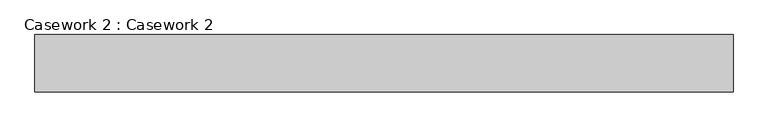
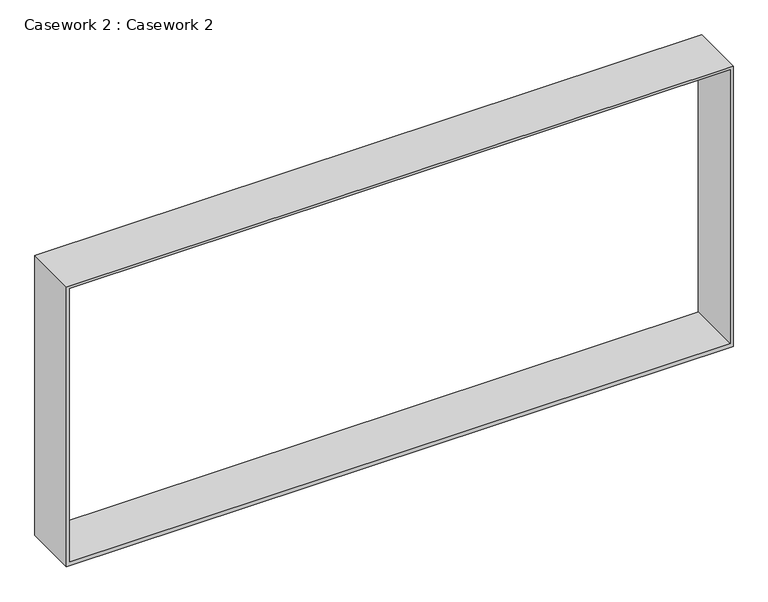
"""IFC4 building model written with IfcOpenShell, lengths in millimetres: furniture geometry, Casework 2 : Casework 2."""

from ifc_helpers import new_model, si_unit, frame, origin, place, context, project, spatial, polyline, outline, extrude, source, transform, mapped, element, save


def casework_2_casework_2_6ee2d2ed(model_context):
    return source(origin(), model_context, "Body", "SweptSolid", [
        extrude(outline(polyline([(3048.0, -51476.762416), (609.6, -51476.762416), (609.6, -45990.362416), (3048.0, -45990.362416), (3048.0, -51476.762416)]), holes=[polyline([(3024.850107, -51451.362416), (3024.850107, -46015.762416), (643.13302, -46015.762416), (643.13302, -51451.362416), (3024.850107, -51451.362416)])]), frame((0.0, 285614.3720148, 0.0), z_axis=(0.0, 1.0, 0.0), x_axis=(0.0, 0.0, 1.0)), (0.0, 0.0, 1.0), 450.1962661),
    ])


if __name__ == "__main__":
    model = new_model("IFC4")
    model_context = context("Model", 3, world=origin())
    ifc_project = project(units=[si_unit("LENGTHUNIT", "METRE", prefix="MILLI")], contexts=[model_context])
    site = spatial("IfcSite", under=ifc_project)
    building = spatial("IfcBuilding", under=site)
    placement = place(None, origin())
    casework_2_casework_2_shape = casework_2_casework_2_6ee2d2ed(model_context)
    element("IfcFurniture", 1, ObjectType="Casework 2 : Casework 2", at=placement, inside=building, context=model_context, shape_type="MappedRepresentation", body=[
        mapped(casework_2_casework_2_shape, transform((0.0, 0.0, 0.0), x_axis=(1.0, 0.0, 0.0), y_axis=(0.0, 1.0, 0.0), z_axis=(0.0, 0.0, 1.0))),
    ])
    save(model, "model.ifc")

# Revit data of these elements
# Element 1 (IfcFurniture, "Casework 2 : Casework 2")
#   Materials on its faces: "Dark metal"
# Materials
#   "Dark metal": class "Generic", colour RGB 44 29 29, transparency 0, Cost = 0
